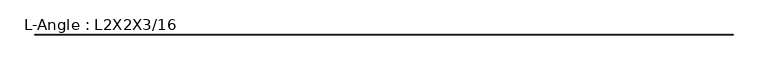
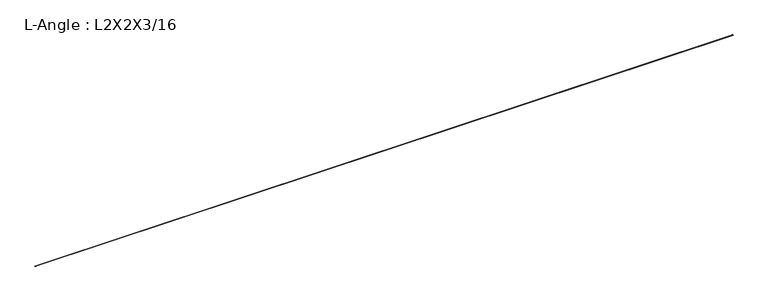
"""IFC4 building model written with IfcOpenShell, lengths in millimetres: beam geometry, L-Angle : L2X2X3/16."""

import ifcopenshell
import ifcopenshell.guid

model = None  # the IFC model being written
_history = None  # IfcOwnerHistory: only IFC2X3 demands one
_inside = {}  # id of a spatial element -> (the spatial element, [elements in it])
_under = {}  # id of a project, library or spatial element -> (it, [spatial elements below it])
_declared = {}  # id of a project -> (the project, [libraries it declares])
_typed = {}  # id of a type object -> (the type object, [elements of that type])
_made_of = {}  # id of a material, layer set ... -> (it, [elements and type objects made of it])


def new_model(schema):
    """Start an empty IFC model of exactly this schema.

    Asked for "IFC4X3", IfcOpenShell would pick the latest addendum, in which some entities
    have other attributes; the version numbers below select the first issue.
    IFC2X3 requires an IfcOwnerHistory on every rooted entity: one is made here for all.
    """
    global model, _history
    if schema == "IFC4X3":
        model = ifcopenshell.file(schema_version=(4, 3, 0, 0))
    else:
        model = ifcopenshell.file(schema=schema)
    _inside.clear()
    _under.clear()
    _declared.clear()
    _typed.clear()
    _made_of.clear()
    _history = None
    if model.schema == "IFC2X3":
        org = make("IfcOrganization", Name="unknown")
        user = make(
            "IfcPersonAndOrganization",
            ThePerson=make("IfcPerson", FamilyName="unknown"),
            TheOrganization=org,
        )
        app = make(
            "IfcApplication",
            ApplicationDeveloper=org,
            Version="unknown",
            ApplicationFullName="unknown",
            ApplicationIdentifier="unknown",
        )
        _history = make(
            "IfcOwnerHistory",
            OwningUser=user,
            OwningApplication=app,
            ChangeAction="ADDED",
            CreationDate=0,
        )
    return model


def make(cls, **values):
    """One entity of the class cls with the attributes given. An attribute that is None is left unset."""
    return model.create_entity(
        cls, **{name: value for name, value in values.items() if value is not None}
    )


def rooted(cls, **values):
    """An entity with a GlobalId (a new one), such as an element, a storey or a relation."""
    return make(cls, GlobalId=ifcopenshell.guid.new(), OwnerHistory=_history, **values)


def si_unit(unit_type, name, prefix=None):
    """IfcSIUnit, for example si_unit("LENGTHUNIT", "METRE", prefix="MILLI")."""
    return make("IfcSIUnit", UnitType=unit_type, Prefix=prefix, Name=name)


def assignment(units):
    """IfcUnitAssignment: the units of a project."""
    return None if units is None else make("IfcUnitAssignment", Units=units)


def point(xyz):
    """IfcCartesianPoint."""
    return None if xyz is None else make("IfcCartesianPoint", Coordinates=xyz)


def direction(xyz):
    """IfcDirection."""
    return None if xyz is None else make("IfcDirection", DirectionRatios=xyz)


def frame(location, z_axis=None, x_axis=None):
    """IfcAxis2Placement3D, a coordinate frame: its origin and axes. An axis left out is left unset."""
    return make(
        "IfcAxis2Placement3D",
        Location=point(location),
        Axis=direction(z_axis),
        RefDirection=direction(x_axis),
    )


def frame_2d(location, x_axis=None):
    """IfcAxis2Placement2D, a coordinate frame in the plane: its origin and x axis."""
    return make(
        "IfcAxis2Placement2D", Location=point(location), RefDirection=direction(x_axis)
    )


def origin():
    """The frame at (0, 0, 0) with its axes left unset."""
    return frame((0.0, 0.0, 0.0))


def place(relative_to, where):
    """IfcLocalPlacement: puts the frame where relative to a parent placement (None: the world)."""
    return make(
        "IfcLocalPlacement", PlacementRelTo=relative_to, RelativePlacement=where
    )


def context(
    kind, dimensions, precision=None, world=None, true_north=None, identifier=None
):
    """IfcGeometricRepresentationContext, for example the 3D "Model" context."""
    return make(
        "IfcGeometricRepresentationContext",
        ContextIdentifier=identifier,
        ContextType=kind,
        CoordinateSpaceDimension=dimensions,
        Precision=precision,
        WorldCoordinateSystem=world,
        TrueNorth=true_north,
    )


def project(units=None, contexts=None):
    """IfcProject with its units and contexts."""
    return rooted(
        "IfcProject",
        Name="project",
        RepresentationContexts=contexts,
        UnitsInContext=assignment(units),
    )


def spatial(cls, under=None, at=None, **own):
    """A site, building, storey or space (cls), placed at a placement, below another one or the project."""
    s = rooted(cls, ObjectPlacement=at, **own)
    if under is not None:
        _under.setdefault(under.id(), (under, []))[1].append(s)
    return s


def polyline(points):
    """IfcPolyline through the points."""
    return make("IfcPolyline", Points=[point(p) for p in points])


def circle_curve(where, radius):
    """IfcCircle in the frame where."""
    return make("IfcCircle", Position=where, Radius=radius)


def trimmed(basis, trim1, trim2, sense, master):
    """IfcTrimmedCurve: the piece of a basis curve between two trims."""
    return make(
        "IfcTrimmedCurve",
        BasisCurve=basis,
        Trim1=trim1,
        Trim2=trim2,
        SenseAgreement=sense,
        MasterRepresentation=master,
    )


def segment(curve, same_sense, transition):
    """IfcCompositeCurveSegment."""
    return make(
        "IfcCompositeCurveSegment",
        Transition=transition,
        SameSense=same_sense,
        ParentCurve=curve,
    )


def composite_curve(segments, self_intersect=None):
    """IfcCompositeCurve: segments joined end to end."""
    return make("IfcCompositeCurve", Segments=segments, SelfIntersect=self_intersect)


def outline(outer, holes=None, kind="AREA"):
    """IfcArbitraryClosedProfileDef: a profile drawn as a closed curve; with holes, ...WithVoids."""
    if holes is None:
        return make("IfcArbitraryClosedProfileDef", ProfileType=kind, OuterCurve=outer)
    return make(
        "IfcArbitraryProfileDefWithVoids",
        ProfileType=kind,
        OuterCurve=outer,
        InnerCurves=holes,
    )


def extrude(swept, where, along, depth):
    """IfcExtrudedAreaSolid: the profile swept, set in the frame where, extruded along a direction by depth."""
    return make(
        "IfcExtrudedAreaSolid",
        SweptArea=swept,
        Position=where,
        ExtrudedDirection=direction(along),
        Depth=depth,
    )


def shape(context_of_items, identifier, shape_type, items):
    """IfcShapeRepresentation: the items that make up one representation, for example the "Body"."""
    return make(
        "IfcShapeRepresentation",
        ContextOfItems=context_of_items,
        RepresentationIdentifier=identifier,
        RepresentationType=shape_type,
        Items=items,
    )


def source(mapping_origin, context_of_items, identifier, shape_type, items):
    """IfcRepresentationMap: a shape defined once, which mapped items show again and again."""
    return make(
        "IfcRepresentationMap",
        MappingOrigin=mapping_origin,
        MappedRepresentation=shape(context_of_items, identifier, shape_type, items),
    )


def transform(
    local_origin,
    x_axis=None,
    y_axis=None,
    z_axis=None,
    scale=None,
    scale2=None,
    scale3=None,
    uniform=True,
):
    """IfcCartesianTransformationOperator3D, or its non-uniform kind. x_axis, y_axis, z_axis: its Axis1, 2, 3."""
    if uniform:
        return make(
            "IfcCartesianTransformationOperator3D",
            Axis1=direction(x_axis),
            Axis2=direction(y_axis),
            LocalOrigin=point(local_origin),
            Scale=scale,
            Axis3=direction(z_axis),
        )
    return make(
        "IfcCartesianTransformationOperator3DnonUniform",
        Axis1=direction(x_axis),
        Axis2=direction(y_axis),
        LocalOrigin=point(local_origin),
        Scale=scale,
        Axis3=direction(z_axis),
        Scale2=scale2,
        Scale3=scale3,
    )


def mapped(mapping_source, mapping_target):
    """IfcMappedItem: shows the shape of a source again, moved by a transform."""
    return make(
        "IfcMappedItem", MappingSource=mapping_source, MappingTarget=mapping_target
    )


def made_of(thing, what):
    """Note that an element or type object is made of a material, layer set ...; save() writes the relation."""
    if what is not None:
        _made_of.setdefault(what.id(), (what, []))[1].append(thing)
    return thing


def element(
    cls,
    number,
    at=None,
    inside=None,
    cuts=None,
    type_object=None,
    material=None,
    context=None,
    identifier="Body",
    shape_type=None,
    held_by="IfcProductDefinitionShape",
    body=None,
    shapes=None,
    **own,
):
    """One element of the class cls, such as IfcWall. Its Tag is "e" and its number.

    at: its placement. inside: the storey or other place that contains it. cuts: it is an
    opening in that element (IfcRelVoidsElement). A single representation is given by context,
    identifier, shape_type and body (its items); several are given by shapes. held_by: the class
    of the entity that holds the representations. save() writes the other relations.
    """
    e = rooted(cls, Tag="e%d" % number, ObjectPlacement=at, **own)
    if body is not None:
        shapes = [shape(context, identifier, shape_type, body)]
    if shapes is not None:
        e.Representation = make(held_by, Representations=shapes)
    if inside is not None:
        _inside.setdefault(inside.id(), (inside, []))[1].append(e)
    if cuts is not None:
        rooted(
            "IfcRelVoidsElement", RelatingBuildingElement=cuts, RelatedOpeningElement=e
        )
    if type_object is not None:
        _typed.setdefault(type_object.id(), (type_object, []))[1].append(e)
    return made_of(e, material)


def aggregate(whole, parts):
    """IfcRelAggregates: a whole, such as a stair, and the parts it consists of."""
    return rooted("IfcRelAggregates", RelatingObject=whole, RelatedObjects=parts)


def save(model, path):
    """Write the relations noted so far, then the file.

    IfcRelAggregates (storeys below a building ...), IfcRelContainedInSpatialStructure (elements
    in a storey), IfcRelDefinesByType, IfcRelAssociatesMaterial and IfcRelDeclares: one each for
    every whole, place, type object, material and project.
    """
    for whole, parts in _under.values():
        aggregate(whole, parts)
    for where, things in _inside.values():
        rooted(
            "IfcRelContainedInSpatialStructure",
            RelatedElements=things,
            RelatingStructure=where,
        )
    for kind, things in _typed.values():
        rooted("IfcRelDefinesByType", RelatedObjects=things, RelatingType=kind)
    for what, things in _made_of.values():
        rooted("IfcRelAssociatesMaterial", RelatedObjects=things, RelatingMaterial=what)
    for by, libraries in _declared.values():
        rooted("IfcRelDeclares", RelatingContext=by, RelatedDefinitions=libraries)
    model.write(path)


def l_angle_l2x2x3_16_cd50c46b(model_context):
    return source(origin(), model_context, "Body", "SweptSolid", [
        extrude(outline(composite_curve([segment(polyline([(14.2494, 14.2494), (14.2494, -36.5506)]), True, "CONTINUOUS"), segment(trimmed(circle_curve(frame_2d((14.2494, -31.7881)), 4.7625), [point((14.2494, -36.5506))], [point((9.4869, -31.7881))], False, "CARTESIAN"), True, "CONTINUOUS"), segment(polyline([(9.4869, -31.7881), (9.4869, 4.7244)]), True, "CONTINUOUS"), segment(trimmed(circle_curve(frame_2d((4.7244, 4.7244)), 4.7625), [point((9.4869, 4.7244))], [point((4.7244, 9.4869))], True, "CARTESIAN"), True, "CONTINUOUS"), segment(polyline([(4.7244, 9.4869), (-31.7881, 9.4869)]), True, "CONTINUOUS"), segment(trimmed(circle_curve(frame_2d((-31.7881, 14.2494)), 4.7625), [point((-31.7881, 9.4869))], [point((-36.5506, 14.2494))], False, "CARTESIAN"), True, "CONTINUOUS"), segment(polyline([(-36.5506, 14.2494), (14.2494, 14.2494)]), True, "CONTINUOUS")], self_intersect=False)), frame((-44323.0, 0.0, 0.0), z_axis=(1.0, 0.0, 0.0), x_axis=(0.0, 1.0, 0.0)), (0.0, 0.0, 1.0), 88430.1),
    ])


if __name__ == "__main__":
    model = new_model("IFC4")
    model_context = context("Model", 3, world=origin())
    ifc_project = project(units=[si_unit("LENGTHUNIT", "METRE", prefix="MILLI")], contexts=[model_context])
    site = spatial("IfcSite", under=ifc_project)
    building = spatial("IfcBuilding", under=site)
    placement = place(None, origin())
    l_angle_l2x2x3_16_shape = l_angle_l2x2x3_16_cd50c46b(model_context)
    element("IfcBeam", 1, ObjectType="L-Angle : L2X2X3/16", at=placement, inside=building, context=model_context, shape_type="MappedRepresentation", body=[
        mapped(l_angle_l2x2x3_16_shape, transform((0.0, 0.0, 0.0), x_axis=(1.0, 0.0, 0.0), y_axis=(0.0, 1.0, 0.0), z_axis=(0.0, 0.0, 1.0))),
    ])
    save(model, "model.ifc")

# Revit data of these elements
# Type "L-Angle : L2X2X3/16"
#   Assembly Code = "B10"
#   k = 0' - 0 7/16"
#   W = 2.44
#   Start Extension Calculation [instance default] = 10' - 0"
#   Start Extension [instance default] = -0' - 0 1/2"
#   End Extension Calculation [instance default] = 10' - 0"
#   End Extension [instance default] = -0' - 0 1/2"
#   Length [instance default] = 5' - 0"
#   b = 0' - 2"
#   d = 0' - 2"
#   t = 0' - 0 3/16"
#   x = 0' - 0.561"
#   y = 0' - 0.561"
#   A = 0.00496528 SF
#   Structural Material [instance default] = Metal - Steel - ASTM A36
# Element 1 (IfcBeam, "L-Angle : L2X2X3/16")
#   Structural Material = STRUCTURAL STEEL - SEE STRUCT. DWGS
#   Materials on its faces: "STRUCTURAL STEEL - SEE STRUCT. DWGS"
# Materials
#   "Metal - Steel - ASTM A36": class "Metal", colour RGB 199 199 199, transparency 0
#   "STRUCTURAL STEEL - SEE STRUCT. DWGS": class "Metal", colour RGB 137 146 153, transparency 0, Description = "Steel, mill finish", Cost = 0
